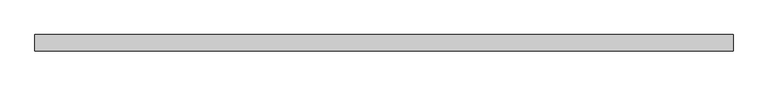
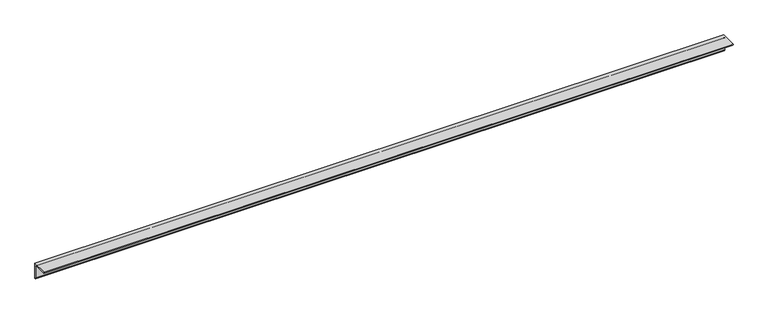
"""IFC4 building model written with IfcOpenShell, lengths in millimetres: member geometry, 0912_Steel Framing_L-KSD3502 : H_SB_AR_S03_L-130x130x12_HBR3."""

import ifcopenshell
import ifcopenshell.guid

model = None  # the IFC model being written
_history = None  # IfcOwnerHistory: only IFC2X3 demands one
_inside = {}  # id of a spatial element -> (the spatial element, [elements in it])
_under = {}  # id of a project, library or spatial element -> (it, [spatial elements below it])
_declared = {}  # id of a project -> (the project, [libraries it declares])
_typed = {}  # id of a type object -> (the type object, [elements of that type])
_made_of = {}  # id of a material, layer set ... -> (it, [elements and type objects made of it])


def new_model(schema):
    """Start an empty IFC model of exactly this schema.

    Asked for "IFC4X3", IfcOpenShell would pick the latest addendum, in which some entities
    have other attributes; the version numbers below select the first issue.
    IFC2X3 requires an IfcOwnerHistory on every rooted entity: one is made here for all.
    """
    global model, _history
    if schema == "IFC4X3":
        model = ifcopenshell.file(schema_version=(4, 3, 0, 0))
    else:
        model = ifcopenshell.file(schema=schema)
    _inside.clear()
    _under.clear()
    _declared.clear()
    _typed.clear()
    _made_of.clear()
    _history = None
    if model.schema == "IFC2X3":
        org = make("IfcOrganization", Name="unknown")
        user = make(
            "IfcPersonAndOrganization",
            ThePerson=make("IfcPerson", FamilyName="unknown"),
            TheOrganization=org,
        )
        app = make(
            "IfcApplication",
            ApplicationDeveloper=org,
            Version="unknown",
            ApplicationFullName="unknown",
            ApplicationIdentifier="unknown",
        )
        _history = make(
            "IfcOwnerHistory",
            OwningUser=user,
            OwningApplication=app,
            ChangeAction="ADDED",
            CreationDate=0,
        )
    return model


def make(cls, **values):
    """One entity of the class cls with the attributes given. An attribute that is None is left unset."""
    return model.create_entity(
        cls, **{name: value for name, value in values.items() if value is not None}
    )


def rooted(cls, **values):
    """An entity with a GlobalId (a new one), such as an element, a storey or a relation."""
    return make(cls, GlobalId=ifcopenshell.guid.new(), OwnerHistory=_history, **values)


def si_unit(unit_type, name, prefix=None):
    """IfcSIUnit, for example si_unit("LENGTHUNIT", "METRE", prefix="MILLI")."""
    return make("IfcSIUnit", UnitType=unit_type, Prefix=prefix, Name=name)


def assignment(units):
    """IfcUnitAssignment: the units of a project."""
    return None if units is None else make("IfcUnitAssignment", Units=units)


def point(xyz):
    """IfcCartesianPoint."""
    return None if xyz is None else make("IfcCartesianPoint", Coordinates=xyz)


def direction(xyz):
    """IfcDirection."""
    return None if xyz is None else make("IfcDirection", DirectionRatios=xyz)


def frame(location, z_axis=None, x_axis=None):
    """IfcAxis2Placement3D, a coordinate frame: its origin and axes. An axis left out is left unset."""
    return make(
        "IfcAxis2Placement3D",
        Location=point(location),
        Axis=direction(z_axis),
        RefDirection=direction(x_axis),
    )


def frame_2d(location, x_axis=None):
    """IfcAxis2Placement2D, a coordinate frame in the plane: its origin and x axis."""
    return make(
        "IfcAxis2Placement2D", Location=point(location), RefDirection=direction(x_axis)
    )


def origin():
    """The frame at (0, 0, 0) with its axes left unset."""
    return frame((0.0, 0.0, 0.0))


def place(relative_to, where):
    """IfcLocalPlacement: puts the frame where relative to a parent placement (None: the world)."""
    return make(
        "IfcLocalPlacement", PlacementRelTo=relative_to, RelativePlacement=where
    )


def context(
    kind, dimensions, precision=None, world=None, true_north=None, identifier=None
):
    """IfcGeometricRepresentationContext, for example the 3D "Model" context."""
    return make(
        "IfcGeometricRepresentationContext",
        ContextIdentifier=identifier,
        ContextType=kind,
        CoordinateSpaceDimension=dimensions,
        Precision=precision,
        WorldCoordinateSystem=world,
        TrueNorth=true_north,
    )


def project(units=None, contexts=None):
    """IfcProject with its units and contexts."""
    return rooted(
        "IfcProject",
        Name="project",
        RepresentationContexts=contexts,
        UnitsInContext=assignment(units),
    )


def spatial(cls, under=None, at=None, **own):
    """A site, building, storey or space (cls), placed at a placement, below another one or the project."""
    s = rooted(cls, ObjectPlacement=at, **own)
    if under is not None:
        _under.setdefault(under.id(), (under, []))[1].append(s)
    return s


def polyline(points):
    """IfcPolyline through the points."""
    return make("IfcPolyline", Points=[point(p) for p in points])


def circle_curve(where, radius):
    """IfcCircle in the frame where."""
    return make("IfcCircle", Position=where, Radius=radius)


def trimmed(basis, trim1, trim2, sense, master):
    """IfcTrimmedCurve: the piece of a basis curve between two trims."""
    return make(
        "IfcTrimmedCurve",
        BasisCurve=basis,
        Trim1=trim1,
        Trim2=trim2,
        SenseAgreement=sense,
        MasterRepresentation=master,
    )


def segment(curve, same_sense, transition):
    """IfcCompositeCurveSegment."""
    return make(
        "IfcCompositeCurveSegment",
        Transition=transition,
        SameSense=same_sense,
        ParentCurve=curve,
    )


def composite_curve(segments, self_intersect=None):
    """IfcCompositeCurve: segments joined end to end."""
    return make("IfcCompositeCurve", Segments=segments, SelfIntersect=self_intersect)


def outline(outer, holes=None, kind="AREA"):
    """IfcArbitraryClosedProfileDef: a profile drawn as a closed curve; with holes, ...WithVoids."""
    if holes is None:
        return make("IfcArbitraryClosedProfileDef", ProfileType=kind, OuterCurve=outer)
    return make(
        "IfcArbitraryProfileDefWithVoids",
        ProfileType=kind,
        OuterCurve=outer,
        InnerCurves=holes,
    )


def extrude(swept, where, along, depth):
    """IfcExtrudedAreaSolid: the profile swept, set in the frame where, extruded along a direction by depth."""
    return make(
        "IfcExtrudedAreaSolid",
        SweptArea=swept,
        Position=where,
        ExtrudedDirection=direction(along),
        Depth=depth,
    )


def shape(context_of_items, identifier, shape_type, items):
    """IfcShapeRepresentation: the items that make up one representation, for example the "Body"."""
    return make(
        "IfcShapeRepresentation",
        ContextOfItems=context_of_items,
        RepresentationIdentifier=identifier,
        RepresentationType=shape_type,
        Items=items,
    )


def source(mapping_origin, context_of_items, identifier, shape_type, items):
    """IfcRepresentationMap: a shape defined once, which mapped items show again and again."""
    return make(
        "IfcRepresentationMap",
        MappingOrigin=mapping_origin,
        MappedRepresentation=shape(context_of_items, identifier, shape_type, items),
    )


def transform(
    local_origin,
    x_axis=None,
    y_axis=None,
    z_axis=None,
    scale=None,
    scale2=None,
    scale3=None,
    uniform=True,
):
    """IfcCartesianTransformationOperator3D, or its non-uniform kind. x_axis, y_axis, z_axis: its Axis1, 2, 3."""
    if uniform:
        return make(
            "IfcCartesianTransformationOperator3D",
            Axis1=direction(x_axis),
            Axis2=direction(y_axis),
            LocalOrigin=point(local_origin),
            Scale=scale,
            Axis3=direction(z_axis),
        )
    return make(
        "IfcCartesianTransformationOperator3DnonUniform",
        Axis1=direction(x_axis),
        Axis2=direction(y_axis),
        LocalOrigin=point(local_origin),
        Scale=scale,
        Axis3=direction(z_axis),
        Scale2=scale2,
        Scale3=scale3,
    )


def mapped(mapping_source, mapping_target):
    """IfcMappedItem: shows the shape of a source again, moved by a transform."""
    return make(
        "IfcMappedItem", MappingSource=mapping_source, MappingTarget=mapping_target
    )


def made_of(thing, what):
    """Note that an element or type object is made of a material, layer set ...; save() writes the relation."""
    if what is not None:
        _made_of.setdefault(what.id(), (what, []))[1].append(thing)
    return thing


def element(
    cls,
    number,
    at=None,
    inside=None,
    cuts=None,
    type_object=None,
    material=None,
    context=None,
    identifier="Body",
    shape_type=None,
    held_by="IfcProductDefinitionShape",
    body=None,
    shapes=None,
    **own,
):
    """One element of the class cls, such as IfcWall. Its Tag is "e" and its number.

    at: its placement. inside: the storey or other place that contains it. cuts: it is an
    opening in that element (IfcRelVoidsElement). A single representation is given by context,
    identifier, shape_type and body (its items); several are given by shapes. held_by: the class
    of the entity that holds the representations. save() writes the other relations.
    """
    e = rooted(cls, Tag="e%d" % number, ObjectPlacement=at, **own)
    if body is not None:
        shapes = [shape(context, identifier, shape_type, body)]
    if shapes is not None:
        e.Representation = make(held_by, Representations=shapes)
    if inside is not None:
        _inside.setdefault(inside.id(), (inside, []))[1].append(e)
    if cuts is not None:
        rooted(
            "IfcRelVoidsElement", RelatingBuildingElement=cuts, RelatedOpeningElement=e
        )
    if type_object is not None:
        _typed.setdefault(type_object.id(), (type_object, []))[1].append(e)
    return made_of(e, material)


def aggregate(whole, parts):
    """IfcRelAggregates: a whole, such as a stair, and the parts it consists of."""
    return rooted("IfcRelAggregates", RelatingObject=whole, RelatedObjects=parts)


def save(model, path):
    """Write the relations noted so far, then the file.

    IfcRelAggregates (storeys below a building ...), IfcRelContainedInSpatialStructure (elements
    in a storey), IfcRelDefinesByType, IfcRelAssociatesMaterial and IfcRelDeclares: one each for
    every whole, place, type object, material and project.
    """
    for whole, parts in _under.values():
        aggregate(whole, parts)
    for where, things in _inside.values():
        rooted(
            "IfcRelContainedInSpatialStructure",
            RelatedElements=things,
            RelatingStructure=where,
        )
    for kind, things in _typed.values():
        rooted("IfcRelDefinesByType", RelatedObjects=things, RelatingType=kind)
    for what, things in _made_of.values():
        rooted("IfcRelAssociatesMaterial", RelatedObjects=things, RelatingMaterial=what)
    for by, libraries in _declared.values():
        rooted("IfcRelDeclares", RelatingContext=by, RelatedDefinitions=libraries)
    model.write(path)


def member_53cbeec2(model_context):
    return source(origin(), model_context, "Body", "SweptSolid", [
        extrude(outline(composite_curve([segment(polyline([(36.4, 36.4), (36.4, -93.6)]), True, "CONTINUOUS"), segment(trimmed(circle_curve(frame_2d((36.4, -81.6)), 12.0), [point((36.4, -93.6))], [point((24.4, -81.6))], False, "CARTESIAN"), True, "CONTINUOUS"), segment(polyline([(24.4, -81.6), (24.4, 12.4)]), True, "CONTINUOUS"), segment(trimmed(circle_curve(frame_2d((12.4, 12.4)), 12.0), [point((24.4, 12.4))], [point((12.4, 24.4))], True, "CARTESIAN"), True, "CONTINUOUS"), segment(polyline([(12.4, 24.4), (-81.6, 24.4)]), True, "CONTINUOUS"), segment(trimmed(circle_curve(frame_2d((-81.6, 36.4)), 12.0), [point((-81.6, 24.4))], [point((-93.6, 36.4))], False, "CARTESIAN"), True, "CONTINUOUS"), segment(polyline([(-93.6, 36.4), (36.4, 36.4)]), True, "CONTINUOUS")], self_intersect=False)), frame((-2753.7999994, 0.0, 0.0), z_axis=(1.0, 0.0, 0.0), x_axis=(0.0, 1.0, 0.0)), (0.0, 0.0, 1.0), 5507.5999988),
    ])


if __name__ == "__main__":
    model = new_model("IFC4")
    model_context = context("Model", 3, world=origin())
    ifc_project = project(units=[si_unit("LENGTHUNIT", "METRE", prefix="MILLI")], contexts=[model_context])
    site = spatial("IfcSite", under=ifc_project)
    building = spatial("IfcBuilding", under=site)
    placement = place(None, origin())
    member_shape = member_53cbeec2(model_context)
    element("IfcMember", 1, ObjectType="0912_Steel Framing_L-KSD3502 : H_SB_AR_S03_L-130x130x12_HBR3", at=placement, inside=building, context=model_context, shape_type="MappedRepresentation", body=[
        mapped(member_shape, transform((0.0, 0.0, 0.0), x_axis=(1.0, 0.0, 0.0), y_axis=(0.0, 1.0, 0.0), z_axis=(0.0, 0.0, 1.0))),
    ])
    save(model, "model.ifc")

# Revit data of these elements
# Type "0912_Steel Framing_L-KSD3502 : H_SB_AR_S03_L-130x130x12_HBR3"
#   k = 25 mm
#   Perimeter = 0.52 m²/m
#   Nominal Weight = 23.40 kgf/m
#   Length [instance default] = 1000 mm
#   b = 130 mm
#   d = 130 mm
#   t = 12 mm
#   x = 36.4 mm
#   y = 36.4 mm
#   A = 2976.00 m²
#   Structural Material [instance default] = Steel, 45-345
# Element 1 (IfcMember, "0912_Steel Framing_L-KSD3502 : H_SB_AR_S03_L-130x130x12_HBR3")
#   Structural Material = Steel ASTM A36
#   Materials on its faces: "Steel ASTM A36"
# Materials
#   "Steel, 45-345": class "Metal", colour RGB 189 187 185, transparency 0, Description = "Steel 345 MPa", Cost = 0
#   "Steel ASTM A36": class "Metal", colour RGB 199 199 199, transparency 0, Description = "Structural steel, ASTM A36 Grade B, mill finish", Cost = 0
